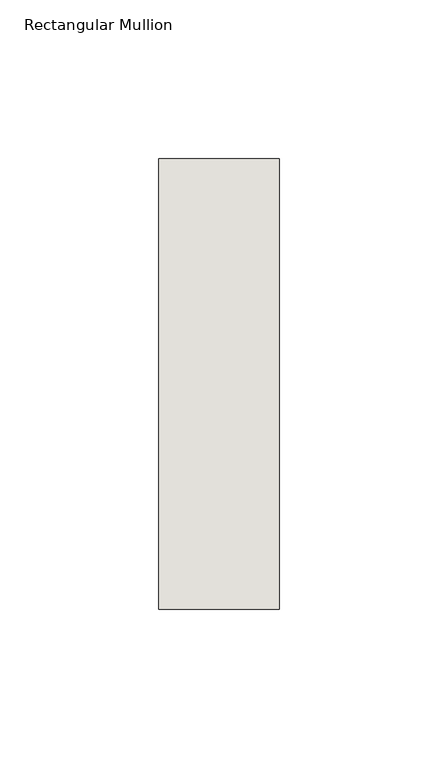
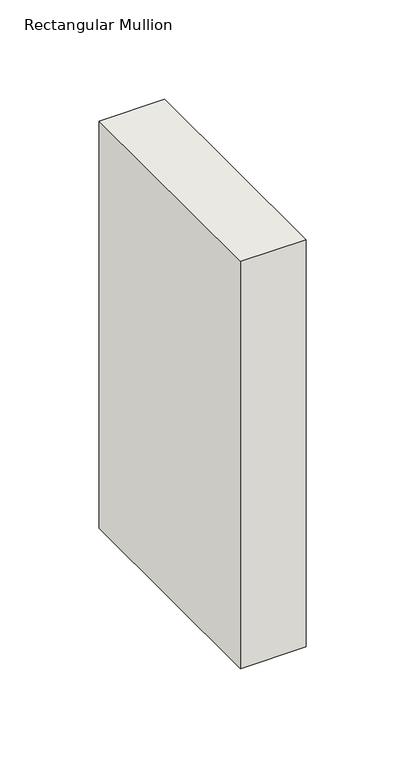
"""IFC4 building model written with IfcOpenShell, lengths in millimetres: wall geometry, Rectangular Mullion : NLRS_21_CWM_hsb-regel 38x142_gen_rsf."""

from ifc_helpers import new_model, si_unit, frame, origin, place, context, project, spatial, polyline, outline, extrude, source, transform, mapped, element, save


def rectangular_mullion_597468ba(model_context):
    return source(origin(), model_context, "Body", "SweptSolid", [
        extrude(outline(polyline([(0.0, -71.0), (-38.0, -71.0), (-38.0, 71.0), (0.0, 71.0), (0.0, -71.0)])), frame((0.0, 0.0, -250.0000003), z_axis=(0.0, 0.0, 1.0), x_axis=(1.0, 0.0, 0.0)), (0.0, 0.0, 1.0), 250.0000003),
    ])


if __name__ == "__main__":
    model = new_model("IFC4")
    model_context = context("Model", 3, world=origin())
    ifc_project = project(units=[si_unit("LENGTHUNIT", "METRE", prefix="MILLI")], contexts=[model_context])
    site = spatial("IfcSite", under=ifc_project)
    building = spatial("IfcBuilding", under=site)
    placement = place(None, origin())
    rectangular_mullion_shape = rectangular_mullion_597468ba(model_context)
    element("IfcWall", 1, ObjectType="Rectangular Mullion : NLRS_21_CWM_hsb-regel 38x142_gen_rsf", at=placement, inside=building, context=model_context, shape_type="MappedRepresentation", body=[
        mapped(rectangular_mullion_shape, transform((0.0, 0.0, 0.0), x_axis=(1.0, 0.0, 0.0), y_axis=(0.0, 1.0, 0.0), z_axis=(0.0, 0.0, 1.0))),
    ])
    save(model, "model.ifc")

# Revit data of these elements
# Type "Rectangular Mullion : NLRS_21_CWM_hsb-regel 38x142_gen_rsf"
#   Type IfcGUID = "07M7mRoiH1CR8m_RSKIwpF"
#   Assembly Code = "21.10"
#   IfcExportAs = "IfcWall"
#   built-in parameter 1007322 = 0.465879 (stored number, unit not read)
#   built-in parameter 1007321 = 0.062336 (stored number, unit not read)
#   built-in parameter 1007320 = 0.062336 (stored number, unit not read)
# Element 1 (IfcWall, "Rectangular Mullion : NLRS_21_CWM_hsb-regel 38x142_gen_rsf")
#   Materials on its faces: "NLRS_i2_hout naaldhout vuren_gen_rsf"
# Materials
#   "NLRS_i2_hout naaldhout vuren_gen_rsf": class "I - Hout", colour RGB 234 199 147, transparency 0, Keynote = "i2", Manufacturer = "Revit Standards Foundation", URL = "www.revitstandards.org", Description = "hout vuren", Cost = 0
